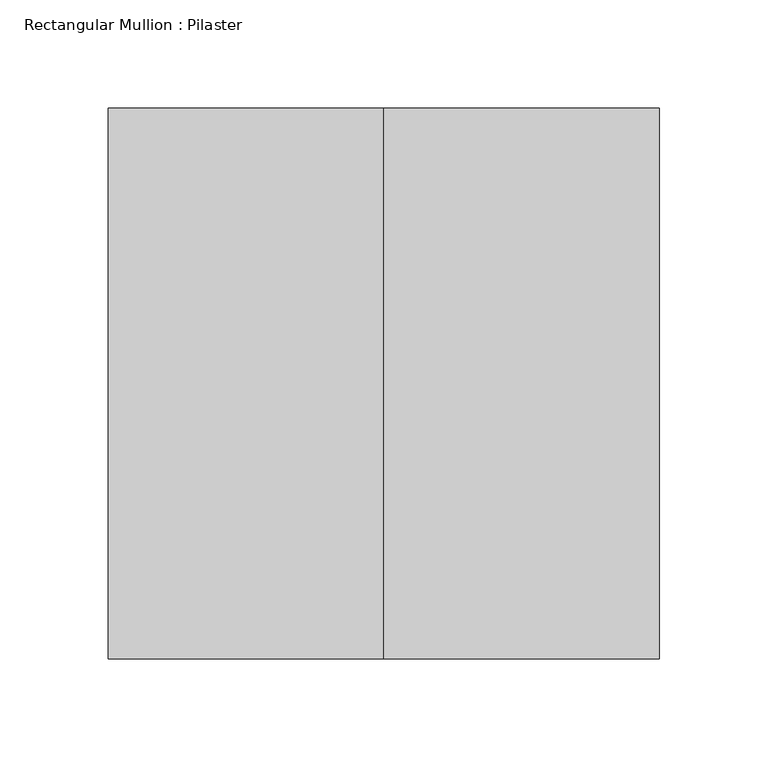
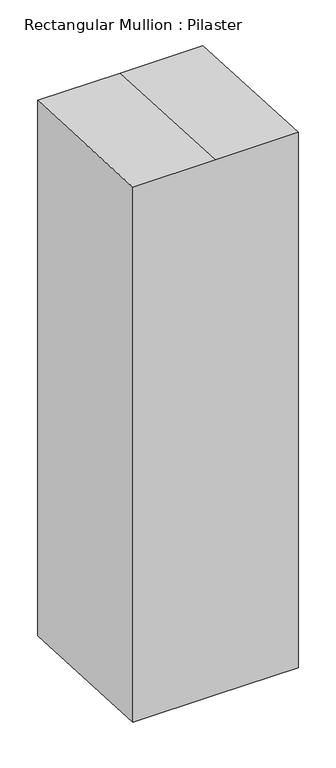
"""IFC4 building model written with IfcOpenShell, lengths in millimetres: member geometry, Rectangular Mullion : Pilaster."""

from ifc_helpers import new_model, si_unit, origin, place, context, project, spatial, faceted_brep, source, transform, mapped, element, save


def rectangular_mullion_pilaster_80411810(model_context):
    return source(origin(), model_context, "Body", "Brep", [
        faceted_brep([(-127.0, 127.0, -2.7320304), (0.0, 127.0, -2.7320304), (127.0, 127.0, -2.7320304), (127.0, 127.0, -872.319055), (0.0, 127.0, -872.319055), (-127.0, 127.0, -872.319055), (-127.0, -127.0, 10.5795456), (-127.0, -127.0, -859.007479), (127.0, -127.0, 10.5795456), (0.0, -127.0, 10.5795456), (0.0, -127.0, -859.007479), (127.0, -127.0, -859.007479)], [[[0, 1, 2, 3, 4, 5]], [[6, 0, 5, 7]], [[8, 9, 6, 7, 10, 11]], [[2, 8, 11, 3]], [[2, 1, 9, 8]], [[1, 0, 6, 9]], [[3, 11, 10, 4]], [[10, 7, 5, 4]]]),
    ])


if __name__ == "__main__":
    model = new_model("IFC4")
    model_context = context("Model", 3, world=origin())
    ifc_project = project(units=[si_unit("LENGTHUNIT", "METRE", prefix="MILLI")], contexts=[model_context])
    site = spatial("IfcSite", under=ifc_project)
    building = spatial("IfcBuilding", under=site)
    placement = place(None, origin())
    rectangular_mullion_pilaster_shape = rectangular_mullion_pilaster_80411810(model_context)
    element("IfcMember", 1, ObjectType="Rectangular Mullion : Pilaster", at=placement, inside=building, context=model_context, shape_type="MappedRepresentation", body=[
        mapped(rectangular_mullion_pilaster_shape, transform((0.0, 0.0, 0.0), x_axis=(1.0, 0.0, 0.0), y_axis=(0.0, 1.0, 0.0), z_axis=(0.0, 0.0, 1.0))),
    ])
    save(model, "model.ifc")

# Revit data of these elements
# Type "Rectangular Mullion : Pilaster"
#   built-in parameter 1007304 = 0.833333 (stored number, unit not read)
#   built-in parameter 1007301 = 0.416667 (stored number, unit not read)
#   built-in parameter 1007300 = 0.416667 (stored number, unit not read)
# Element 1 (IfcMember, "Rectangular Mullion : Pilaster")
#   Materials on its faces: "Aluminum"
# Materials
#   "Aluminum": class "Metal", colour RGB 247 247 247, transparency 0, Description = "Aluminum 6061", Cost = 0
